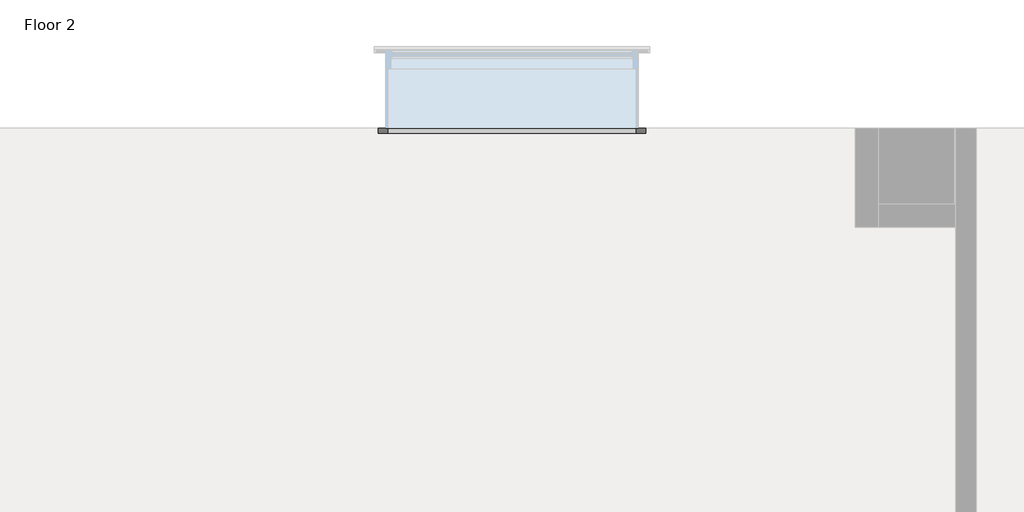
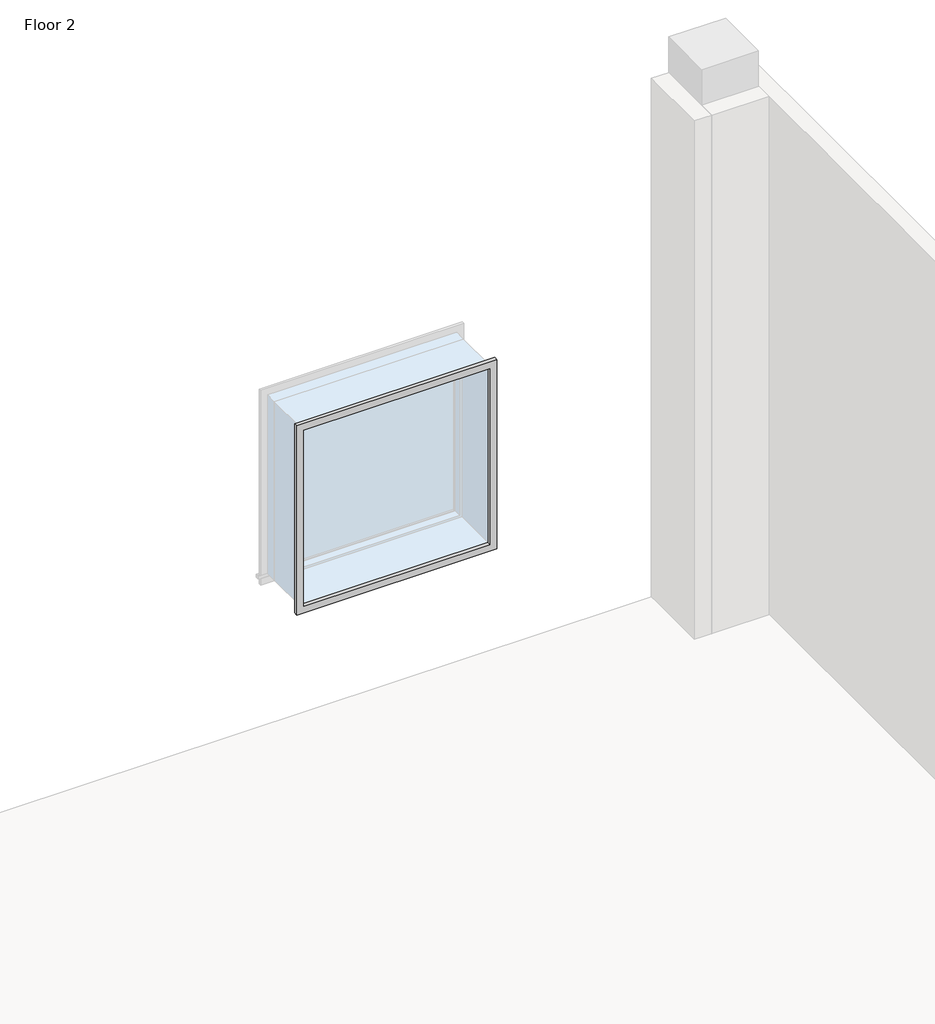
# One storey, part 7 of 7: 1 proxy.
"""IFC4 building model written with IfcOpenShell, lengths in millimetres."""

import ifcopenshell
import ifcopenshell.guid

model = None  # the IFC model being written
_history = None  # IfcOwnerHistory: only IFC2X3 demands one
_inside = {}  # id of a spatial element -> (the spatial element, [elements in it])
_under = {}  # id of a project, library or spatial element -> (it, [spatial elements below it])
_declared = {}  # id of a project -> (the project, [libraries it declares])
_typed = {}  # id of a type object -> (the type object, [elements of that type])
_made_of = {}  # id of a material, layer set ... -> (it, [elements and type objects made of it])


def new_model(schema):
    """Start an empty IFC model of exactly this schema.

    Asked for "IFC4X3", IfcOpenShell would pick the latest addendum, in which some entities
    have other attributes; the version numbers below select the first issue.
    IFC2X3 requires an IfcOwnerHistory on every rooted entity: one is made here for all.
    """
    global model, _history
    if schema == "IFC4X3":
        model = ifcopenshell.file(schema_version=(4, 3, 0, 0))
    else:
        model = ifcopenshell.file(schema=schema)
    _inside.clear()
    _under.clear()
    _declared.clear()
    _typed.clear()
    _made_of.clear()
    _history = None
    if model.schema == "IFC2X3":
        org = make("IfcOrganization", Name="unknown")
        user = make(
            "IfcPersonAndOrganization",
            ThePerson=make("IfcPerson", FamilyName="unknown"),
            TheOrganization=org,
        )
        app = make(
            "IfcApplication",
            ApplicationDeveloper=org,
            Version="unknown",
            ApplicationFullName="unknown",
            ApplicationIdentifier="unknown",
        )
        _history = make(
            "IfcOwnerHistory",
            OwningUser=user,
            OwningApplication=app,
            ChangeAction="ADDED",
            CreationDate=0,
        )
    return model


def make(cls, **values):
    """One entity of the class cls with the attributes given. An attribute that is None is left unset."""
    return model.create_entity(
        cls, **{name: value for name, value in values.items() if value is not None}
    )


def rooted(cls, **values):
    """An entity with a GlobalId (a new one), such as an element, a storey or a relation."""
    return make(cls, GlobalId=ifcopenshell.guid.new(), OwnerHistory=_history, **values)


def si_unit(unit_type, name, prefix=None):
    """IfcSIUnit, for example si_unit("LENGTHUNIT", "METRE", prefix="MILLI")."""
    return make("IfcSIUnit", UnitType=unit_type, Prefix=prefix, Name=name)


def assignment(units):
    """IfcUnitAssignment: the units of a project."""
    return None if units is None else make("IfcUnitAssignment", Units=units)


def point(xyz):
    """IfcCartesianPoint."""
    return None if xyz is None else make("IfcCartesianPoint", Coordinates=xyz)


def direction(xyz):
    """IfcDirection."""
    return None if xyz is None else make("IfcDirection", DirectionRatios=xyz)


def frame(location, z_axis=None, x_axis=None):
    """IfcAxis2Placement3D, a coordinate frame: its origin and axes. An axis left out is left unset."""
    return make(
        "IfcAxis2Placement3D",
        Location=point(location),
        Axis=direction(z_axis),
        RefDirection=direction(x_axis),
    )


def origin():
    """The frame at (0, 0, 0) with its axes left unset."""
    return frame((0.0, 0.0, 0.0))


def origin_with_axes():
    """The frame at (0, 0, 0) with the z axis (0, 0, 1) and the x axis (1, 0, 0) written out."""
    return frame((0.0, 0.0, 0.0), z_axis=(0.0, 0.0, 1.0), x_axis=(1.0, 0.0, 0.0))


def place(relative_to, where):
    """IfcLocalPlacement: puts the frame where relative to a parent placement (None: the world)."""
    return make(
        "IfcLocalPlacement", PlacementRelTo=relative_to, RelativePlacement=where
    )


def context(
    kind, dimensions, precision=None, world=None, true_north=None, identifier=None
):
    """IfcGeometricRepresentationContext, for example the 3D "Model" context."""
    return make(
        "IfcGeometricRepresentationContext",
        ContextIdentifier=identifier,
        ContextType=kind,
        CoordinateSpaceDimension=dimensions,
        Precision=precision,
        WorldCoordinateSystem=world,
        TrueNorth=true_north,
    )


def project(units=None, contexts=None):
    """IfcProject with its units and contexts."""
    return rooted(
        "IfcProject",
        Name="project",
        RepresentationContexts=contexts,
        UnitsInContext=assignment(units),
    )


def spatial(cls, under=None, at=None, **own):
    """A site, building, storey or space (cls), placed at a placement, below another one or the project."""
    s = rooted(cls, ObjectPlacement=at, **own)
    if under is not None:
        _under.setdefault(under.id(), (under, []))[1].append(s)
    return s


def polyline(points):
    """IfcPolyline through the points."""
    return make("IfcPolyline", Points=[point(p) for p in points])


def outline(outer, holes=None, kind="AREA"):
    """IfcArbitraryClosedProfileDef: a profile drawn as a closed curve; with holes, ...WithVoids."""
    if holes is None:
        return make("IfcArbitraryClosedProfileDef", ProfileType=kind, OuterCurve=outer)
    return make(
        "IfcArbitraryProfileDefWithVoids",
        ProfileType=kind,
        OuterCurve=outer,
        InnerCurves=holes,
    )


def extrude(swept, where, along, depth):
    """IfcExtrudedAreaSolid: the profile swept, set in the frame where, extruded along a direction by depth."""
    return make(
        "IfcExtrudedAreaSolid",
        SweptArea=swept,
        Position=where,
        ExtrudedDirection=direction(along),
        Depth=depth,
    )


def shape(context_of_items, identifier, shape_type, items):
    """IfcShapeRepresentation: the items that make up one representation, for example the "Body"."""
    return make(
        "IfcShapeRepresentation",
        ContextOfItems=context_of_items,
        RepresentationIdentifier=identifier,
        RepresentationType=shape_type,
        Items=items,
    )


def source(mapping_origin, context_of_items, identifier, shape_type, items):
    """IfcRepresentationMap: a shape defined once, which mapped items show again and again."""
    return make(
        "IfcRepresentationMap",
        MappingOrigin=mapping_origin,
        MappedRepresentation=shape(context_of_items, identifier, shape_type, items),
    )


def transform(
    local_origin,
    x_axis=None,
    y_axis=None,
    z_axis=None,
    scale=None,
    scale2=None,
    scale3=None,
    uniform=True,
):
    """IfcCartesianTransformationOperator3D, or its non-uniform kind. x_axis, y_axis, z_axis: its Axis1, 2, 3."""
    if uniform:
        return make(
            "IfcCartesianTransformationOperator3D",
            Axis1=direction(x_axis),
            Axis2=direction(y_axis),
            LocalOrigin=point(local_origin),
            Scale=scale,
            Axis3=direction(z_axis),
        )
    return make(
        "IfcCartesianTransformationOperator3DnonUniform",
        Axis1=direction(x_axis),
        Axis2=direction(y_axis),
        LocalOrigin=point(local_origin),
        Scale=scale,
        Axis3=direction(z_axis),
        Scale2=scale2,
        Scale3=scale3,
    )


def mapped(mapping_source, mapping_target):
    """IfcMappedItem: shows the shape of a source again, moved by a transform."""
    return make(
        "IfcMappedItem", MappingSource=mapping_source, MappingTarget=mapping_target
    )


def made_of(thing, what):
    """Note that an element or type object is made of a material, layer set ...; save() writes the relation."""
    if what is not None:
        _made_of.setdefault(what.id(), (what, []))[1].append(thing)
    return thing


def element(
    cls,
    number,
    at=None,
    inside=None,
    cuts=None,
    type_object=None,
    material=None,
    context=None,
    identifier="Body",
    shape_type=None,
    held_by="IfcProductDefinitionShape",
    body=None,
    shapes=None,
    **own,
):
    """One element of the class cls, such as IfcWall. Its Tag is "e" and its number.

    at: its placement. inside: the storey or other place that contains it. cuts: it is an
    opening in that element (IfcRelVoidsElement). A single representation is given by context,
    identifier, shape_type and body (its items); several are given by shapes. held_by: the class
    of the entity that holds the representations. save() writes the other relations.
    """
    e = rooted(cls, Tag="e%d" % number, ObjectPlacement=at, **own)
    if body is not None:
        shapes = [shape(context, identifier, shape_type, body)]
    if shapes is not None:
        e.Representation = make(held_by, Representations=shapes)
    if inside is not None:
        _inside.setdefault(inside.id(), (inside, []))[1].append(e)
    if cuts is not None:
        rooted(
            "IfcRelVoidsElement", RelatingBuildingElement=cuts, RelatedOpeningElement=e
        )
    if type_object is not None:
        _typed.setdefault(type_object.id(), (type_object, []))[1].append(e)
    return made_of(e, material)


def aggregate(whole, parts):
    """IfcRelAggregates: a whole, such as a stair, and the parts it consists of."""
    return rooted("IfcRelAggregates", RelatingObject=whole, RelatedObjects=parts)


def save(model, path):
    """Write the relations noted so far, then the file.

    IfcRelAggregates (storeys below a building ...), IfcRelContainedInSpatialStructure (elements
    in a storey), IfcRelDefinesByType, IfcRelAssociatesMaterial and IfcRelDeclares: one each for
    every whole, place, type object, material and project.
    """
    for whole, parts in _under.values():
        aggregate(whole, parts)
    for where, things in _inside.values():
        rooted(
            "IfcRelContainedInSpatialStructure",
            RelatedElements=things,
            RelatingStructure=where,
        )
    for kind, things in _typed.values():
        rooted("IfcRelDefinesByType", RelatedObjects=things, RelatingType=kind)
    for what, things in _made_of.values():
        rooted("IfcRelAssociatesMaterial", RelatedObjects=things, RelatingMaterial=what)
    for by, libraries in _declared.values():
        rooted("IfcRelDeclares", RelatingContext=by, RelatedDefinitions=libraries)
    model.write(path)


def trim_window_interior_flat_picture_frame_a1a3bc7c(model_context):
    return source(origin(), model_context, "Body", "SweptSolid", [
        extrude(outline(polyline([(806.45, 44.45), (806.45, -1568.45), (-806.45, -1568.45), (-806.45, 44.45), (806.45, 44.45)]), holes=[polyline([(749.3, -12.7), (-749.3, -12.7), (-749.3, -1511.3), (749.3, -1511.3), (749.3, -12.7)])]), origin_with_axes(), (0.0, 0.0, 1.0), 31.75),
    ])


model = new_model("IFC4")

# Units and contexts
model_context = context("Model", 3, world=origin())
ifc_project = project(units=[si_unit("LENGTHUNIT", "METRE", prefix="MILLI")], contexts=[model_context])

# Site, building, storey
site = spatial("IfcSite", under=ifc_project)
building = spatial("IfcBuilding", under=site)
storey = spatial("IfcBuildingStorey", under=building, Name="Floor 2", Elevation=5486.4)

# Proxy
placement = place(None, origin())
trim_window_interior_flat_picture_frame_shape = trim_window_interior_flat_picture_frame_a1a3bc7c(model_context)
element("IfcBuildingElementProxy", 1, Name="Trim-Window-Interior-Flat : Picture Frame", ObjectType="Trim-Window-Interior-Flat : Picture Frame", at=placement, inside=storey, context=model_context, shape_type="MappedRepresentation", body=[
    mapped(trim_window_interior_flat_picture_frame_shape, transform((49690.3692024, 57366.699389, 7924.8), x_axis=(1.0, 0.0, 0.0), y_axis=(0.0, 0.0, 1.0), z_axis=(0.0, -1.0, 0.0))),
])

save(model, "model.ifc")

# Revit data of these elements
# Type "Trim-Window-Interior-Flat : Picture Frame"
#   Trim Thickness_Picture Frame = 0' - 1 1/4"
#   Trim Width = 0' - 2 1/4"
#   Trim Thickness_with Sill = 0' - 0 3/4"
#   Sill Thickness = 0' - 1 1/4"
#   Opening Width [instance default] = 2' - 0"
#   Opening Height [instance default] = 3' - 0"
#   Default Elevation = 4' - 0"
#   Sill = no
#   Picture Frame = yes
#   Trim Material [instance default] = none
# Element 1 (IfcBuildingElementProxy, "Trim-Window-Interior-Flat : Picture Frame")
#   Opening Width = 5' - 0"
#   Opening Height = 5' - 0"
#   Trim Material = Wood - Stained
#   Phase Created = New Construction
#   Materials on its faces: "Wood - Stained"
# Materials
#   "Wood - Stained": class "Wood", colour RGB 224 178 126, transparency 0, Cost = 0
# Area at (36976.793, 53698.224) mm, upper offset 8' - 0", lower offset 0' - 0"
#   Number = "11"
#   Name = "Office Space"
# Area at (9278.212, 48979.66) mm, upper offset 8' - 0", lower offset 0' - 0"
#   Number = "12"
#   Name = "Circulation"
# Area at (6336.769, 21587.48) mm, upper offset 8' - 0", lower offset 0' - 0"
#   Number = "13"
#   Name = "Office Space"
# Area at (1679.486, 48979.66) mm, upper offset 8' - 0", lower offset 0' - 0"
#   Number = "14"
#   Name = "Core"
# Area at (-21668.212, 48979.66) mm, upper offset 8' - 0", lower offset 0' - 0"
#   Number = "15"
#   Name = "Atrium"
# Area at (-5211.968, 48979.66) mm, upper offset 8' - 0", lower offset 0' - 0"
#   Number = "16"
#   Name = "Circulation"
# Area at (49285.761, 46490.382) mm, upper offset 8' - 0", lower offset 0' - 0"
#   Number = "17"
#   Name = "Core"
